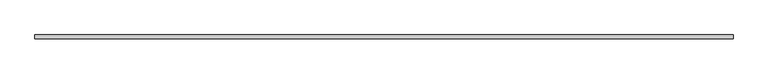
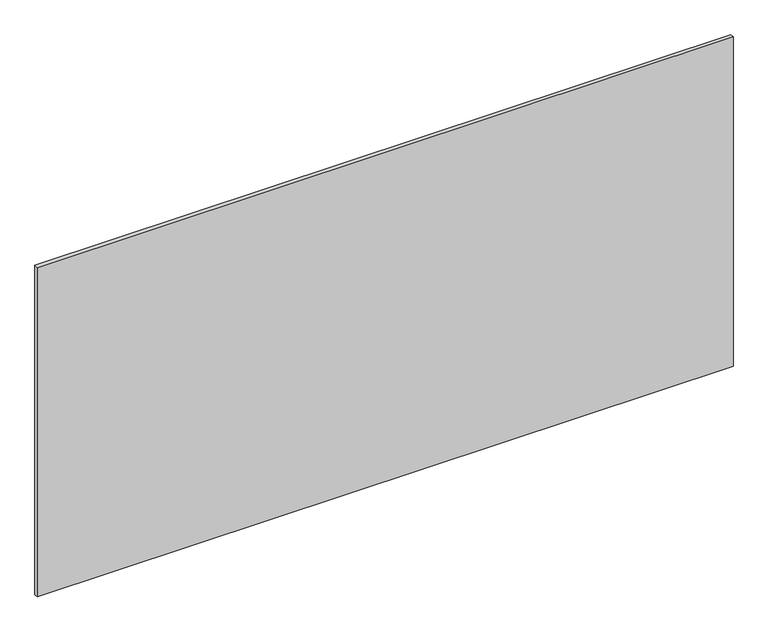
"""IFC4 building model written with IfcOpenShell, lengths in millimetres: proxy geometry, Inner panel:Inner panel:1:Inner panel:1 : Inner panel:Inner panel:300324:300043:Inner panel:1:Inner panel:1 : Inner panel:Inner panel:300324:300043 : Inner panel:Inner panel:1:Inner panel:1 : Inner panel:Inner panel:300324:300043:28 : Inner panel:Inner panel:1:Inner panel:1 : Inner panel:Inner panel:300324:300043:Inner panel:1:Inner panel:1 : Inner panel:Inner panel:300324:300043 : Inner panel:Inner panel:1:Inner panel:1 : Inner panel:Inner panel:300324:300043:300031."""

from ifc_helpers import new_model, si_unit, frame, origin, place, context, project, spatial, polyline, outline, extrude, source, transform, mapped, element, save


def generic_models_991f2966(model_context):
    return source(origin(), model_context, "Body", "SweptSolid", [
        extrude(outline(polyline([(593738.0867239, -579000.6913841), (596176.4867239, -579000.6913841), (596176.4867239, -579013.3913841), (593738.0867239, -579013.3913841), (593738.0867239, -579000.6913841)])), frame((0.0, 0.0, 44.45), z_axis=(0.0, 0.0, 1.0), x_axis=(1.0, 0.0, 0.0)), (0.0, 0.0, 1.0), 1219.2),
    ])


if __name__ == "__main__":
    model = new_model("IFC4")
    model_context = context("Model", 3, world=origin())
    ifc_project = project(units=[si_unit("LENGTHUNIT", "METRE", prefix="MILLI")], contexts=[model_context])
    site = spatial("IfcSite", under=ifc_project)
    building = spatial("IfcBuilding", under=site)
    placement = place(None, origin())
    generic_models_shape = generic_models_991f2966(model_context)
    element("IfcBuildingElementProxy", 1, Name="Inner panel:Inner panel:1:Inner panel:1 : Inner panel:Inner panel:300324:300043:Inner panel:1:Inner panel:1 : Inner panel:Inner panel:300324:300043 : Inner panel:Inner panel:1:Inner panel:1 : Inner panel:Inner panel:300324:300043:28 : Inner panel:Inner panel:1:Inner panel:1 : Inner panel:Inner panel:300324:300043:Inner panel:1:Inner panel:1 : Inner panel:Inner panel:300324:300043 : Inner panel:Inner panel:1:Inner panel:1 : Inner panel:Inner panel:300324:300043:300031", ObjectType="Inner panel:Inner panel:1:Inner panel:1 : Inner panel:Inner panel:300324:300043:Inner panel:1:Inner panel:1 : Inner panel:Inner panel:300324:300043 : Inner panel:Inner panel:1:Inner panel:1 : Inner panel:Inner panel:300324:300043:28 : Inner panel:Inner panel:1:Inner panel:1 : Inner panel:Inner panel:300324:300043:Inner panel:1:Inner panel:1 : Inner panel:Inner panel:300324:300043 : Inner panel:Inner panel:1:Inner panel:1 : Inner panel:Inner panel:300324:300043:300031", at=placement, inside=building, context=model_context, shape_type="MappedRepresentation", body=[
        mapped(generic_models_shape, transform((0.0, 0.0, 0.0), x_axis=(1.0, 0.0, 0.0), y_axis=(0.0, 1.0, 0.0), z_axis=(0.0, 0.0, 1.0))),
    ])
    save(model, "model.ifc")

# Revit data of these elements
# Type "Inner panel:Inner panel:1:Inner panel:1 : Inner panel:Inner panel:300324:300043:Inner panel:1:Inner panel:1 : Inner panel:Inner panel:300324:300043 : Inner panel:Inner panel:1:Inner panel:1 : Inner panel:Inner panel:300324:300043:28 : Inner panel:Inner panel:1:Inner panel:1 : Inner panel:Inner panel:300324:300043:Inner panel:1:Inner panel:1 : Inner panel:Inner panel:300324:300043 : Inner panel:Inner panel:1:Inner panel:1 : Inner panel:Inner panel:300324:300043:300031"
#   NameOverride = "Inner panel:Inner panel:1:Inner panel:1 : Inner panel:Inner panel:300324:300043:Inner panel:1:Inner panel:1 : Inner panel:Inner panel:300324:300043 : Inner panel:Inner panel:1:Inner panel:1 : Inner panel:Inner panel:300324:300043:300031"
#   ObjectTypeOverride = "Inner panel:1:Inner panel:1 : Inner panel:Inner panel:300324:300043 : Inner panel:Inner panel:1:Inner panel:1 : Inner panel:Inner panel:300324:300043"
#   Reference = "Inner panel"
#   Tag = "300031"
# Element 1 (IfcBuildingElementProxy, "Inner panel:Inner panel:1:Inner panel:1 : Inner panel:Inner panel:300324:300043:Inner panel:1:Inner panel:1 : Inner panel:Inner panel:300324:300043 : Inner panel:Inner panel:1:Inner panel:1 : Inner panel:Inner panel:300324:300043:28 : Inner panel:Inner panel:1:Inner panel:1 : Inner panel:Inner panel:300324:300043:Inner panel:1:Inner panel:1 : Inner panel:Inner panel:300324:300043 : Inner panel:Inner panel:1:Inner panel:1 : Inner panel:Inner panel:300324:300043:300031")
#   Materials on its faces: "1/2\" EXTERIOR GRADE FIRE RETARDANT CDX PLYWOOD"
# Materials
#   "1/2\" EXTERIOR GRADE FIRE RETARDANT CDX PLYWOOD": class "Unassigned", colour RGB 196 177 123, transparency 0, Cost = 0
